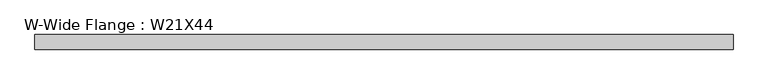
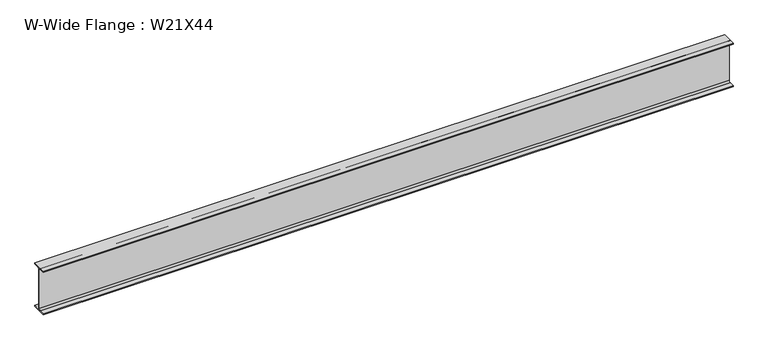
"""IFC4 building model written with IfcOpenShell, lengths in millimetres: beam geometry, W-Wide Flange : W21X44."""

from ifc_helpers import new_model, si_unit, point, frame, frame_2d, origin, place, context, project, spatial, polyline, circle_curve, trimmed, segment, composite_curve, outline, extrude, source, transform, mapped, element, save


def w_wide_flange_w21x44_bf9ef094(model_context):
    return source(origin(), model_context, "Body", "SweptSolid", [
        extrude(outline(composite_curve([segment(polyline([(82.55, -251.46), (82.55, -262.89), (-82.55, -262.89), (-82.55, -251.46), (-21.59, -251.46)]), True, "CONTINUOUS"), segment(trimmed(circle_curve(frame_2d((-21.59, -234.315)), 17.145), [point((-21.59, -251.46))], [point((-4.445, -234.315))], True, "CARTESIAN"), True, "CONTINUOUS"), segment(polyline([(-4.445, -234.315), (-4.445, 234.315)]), True, "CONTINUOUS"), segment(trimmed(circle_curve(frame_2d((-21.59, 234.315)), 17.145), [point((-4.445, 234.315))], [point((-21.59, 251.46))], True, "CARTESIAN"), True, "CONTINUOUS"), segment(polyline([(-21.59, 251.46), (-82.55, 251.46), (-82.55, 262.89), (82.55, 262.89), (82.55, 251.46), (21.59, 251.46)]), True, "CONTINUOUS"), segment(trimmed(circle_curve(frame_2d((21.59, 234.315)), 17.145), [point((21.59, 251.46))], [point((4.445, 234.315))], True, "CARTESIAN"), True, "CONTINUOUS"), segment(polyline([(4.445, 234.315), (4.445, -234.315)]), True, "CONTINUOUS"), segment(trimmed(circle_curve(frame_2d((21.59, -234.315)), 17.145), [point((4.445, -234.315))], [point((21.59, -251.46))], True, "CARTESIAN"), True, "CONTINUOUS"), segment(polyline([(21.59, -251.46), (82.55, -251.46)]), True, "CONTINUOUS")], self_intersect=False)), frame((-3909.0221042, 0.0, 0.0), z_axis=(1.0, 0.0, 0.0), x_axis=(0.0, 1.0, 0.0)), (0.0, 0.0, 1.0), 7878.6241146),
    ])


if __name__ == "__main__":
    model = new_model("IFC4")
    model_context = context("Model", 3, world=origin())
    ifc_project = project(units=[si_unit("LENGTHUNIT", "METRE", prefix="MILLI")], contexts=[model_context])
    site = spatial("IfcSite", under=ifc_project)
    building = spatial("IfcBuilding", under=site)
    placement = place(None, origin())
    w_wide_flange_w21x44_shape = w_wide_flange_w21x44_bf9ef094(model_context)
    element("IfcBeam", 1, ObjectType="W-Wide Flange : W21X44", at=placement, inside=building, context=model_context, shape_type="MappedRepresentation", body=[
        mapped(w_wide_flange_w21x44_shape, transform((0.0, 0.0, 0.0), x_axis=(1.0, 0.0, 0.0), y_axis=(0.0, 1.0, 0.0), z_axis=(0.0, 0.0, 1.0))),
    ])
    save(model, "model.ifc")

# Revit data of these elements
# Type "W-Wide Flange : W21X44"
#   Assembly Code = "B10"
#   W = 44
#   Length [instance default] = 1524 mm
#   bf = 165.1 mm
#   d = 525.78 mm
#   k = 28.575 mm
#   k2 = 17.145 mm
#   tf = 11.43 mm
#   tw = 8.89 mm
#   A = 0.00838708 m²
#   Structural Material [instance default] = Steel ASTM A992
# Element 1 (IfcBeam, "W-Wide Flange : W21X44")
#   Structural Material = Aluminum, Anodized Red
#   Materials on its faces: "Aluminum, Anodized Red"
# Materials
#   "Steel ASTM A992": class "Metal", colour RGB 128 0 0, transparency 0, Description = "Structural steel 50ksi", Cost = 0
#   "Aluminum, Anodized Red": class "Metal", colour RGB 120 120 120, transparency 0, Description = "Anodized aluminum, red", Cost = 0
